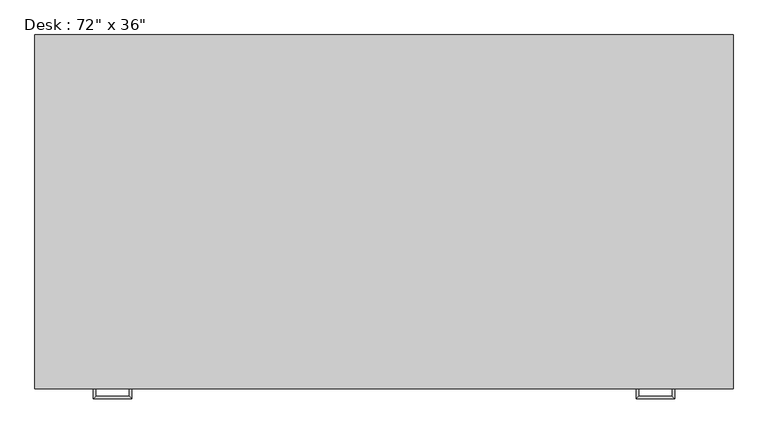
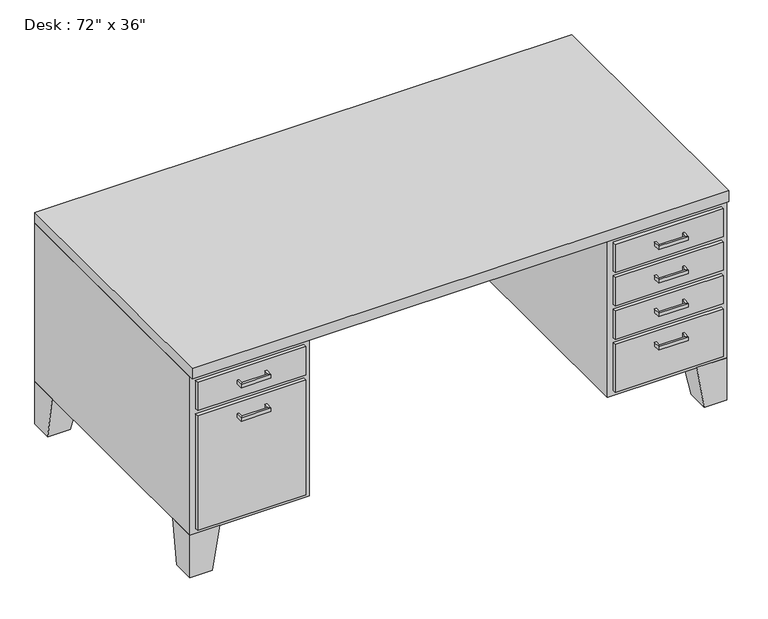
"""IFC4 building model written with IfcOpenShell, lengths in millimetres: furniture geometry."""

from ifc_helpers import new_model, si_unit, frame, origin, place, context, project, spatial, polyline, outline, extrude, faceted_brep, source, transform, mapped, element, save


def furniture_33f25304(model_context):
    return source(origin(), model_context, "Body", "SolidModel", [
        extrude(outline(polyline([(-133.35, -76.2), (234.95, -76.2), (234.95, -88.9), (-133.35, -88.9), (-133.35, -76.2)])), frame((0.0, 0.0, 603.25), z_axis=(0.0, 0.0, 1.0), x_axis=(1.0, 0.0, 0.0)), (0.0, 0.0, 1.0), 101.6),
        extrude(outline(polyline([(-133.35, -76.2), (234.95, -76.2), (234.95, -88.9), (-133.35, -88.9), (-133.35, -76.2)])), frame((0.0, 0.0, 171.45), z_axis=(0.0, 0.0, 1.0), x_axis=(1.0, 0.0, 0.0)), (0.0, 0.0, 1.0), 412.75),
        extrude(outline(polyline([(1289.05, -76.2), (1657.35, -76.2), (1657.35, -88.9), (1289.05, -88.9), (1289.05, -76.2)])), frame((0.0, 0.0, 603.25), z_axis=(0.0, 0.0, 1.0), x_axis=(1.0, 0.0, 0.0)), (0.0, 0.0, 1.0), 101.6),
        extrude(outline(polyline([(1289.05, -76.2), (1657.35, -76.2), (1657.35, -88.9), (1289.05, -88.9), (1289.05, -76.2)])), frame((0.0, 0.0, 171.45), z_axis=(0.0, 0.0, 1.0), x_axis=(1.0, 0.0, 0.0)), (0.0, 0.0, 1.0), 171.45),
        extrude(outline(polyline([(1289.05, -76.2), (1657.35, -76.2), (1657.35, -88.9), (1289.05, -88.9), (1289.05, -76.2)])), frame((0.0, 0.0, 482.6), z_axis=(0.0, 0.0, 1.0), x_axis=(1.0, 0.0, 0.0)), (0.0, 0.0, 1.0), 101.6),
        extrude(outline(polyline([(1289.05, -76.2), (1657.35, -76.2), (1657.35, -88.9), (1289.05, -88.9), (1289.05, -76.2)])), frame((0.0, 0.0, 361.95), z_axis=(0.0, 0.0, 1.0), x_axis=(1.0, 0.0, 0.0)), (0.0, 0.0, 1.0), 101.6),
        faceted_brep([(-50.8, -76.2, 152.4), (-50.8, 25.4, 152.4), (-152.4, 25.4, 152.4), (-152.4, -76.2, 152.4), (-76.2, -76.2, 0.0), (-152.4, -76.2, 0.0), (-152.4, 0.0, 0.0), (-76.2, 0.0, 0.0)], [[[0, 1, 2, 3]], [[4, 5, 6, 7]], [[4, 7, 1, 0]], [[7, 6, 2, 1]], [[6, 5, 3, 2]], [[5, 4, 0, 3]]]),
        faceted_brep([(-50.8, 838.2, 152.4), (-152.4, 838.2, 152.4), (-152.4, 736.6, 152.4), (-50.8, 736.6, 152.4), (-76.2, 838.2, 0.0), (-76.2, 762.0, 0.0), (-152.4, 762.0, 0.0), (-152.4, 838.2, 0.0)], [[[0, 1, 2, 3]], [[4, 5, 6, 7]], [[4, 7, 1, 0]], [[7, 6, 2, 1]], [[6, 5, 3, 2]], [[5, 4, 0, 3]]]),
        faceted_brep([(1574.8, 838.2, 152.4), (1574.8, 736.6, 152.4), (1676.4, 736.6, 152.4), (1676.4, 838.2, 152.4), (1600.2, 838.2, 0.0), (1676.4, 838.2, 0.0), (1676.4, 762.0, 0.0), (1600.2, 762.0, 0.0)], [[[0, 1, 2, 3]], [[4, 5, 6, 7]], [[4, 7, 1, 0]], [[7, 6, 2, 1]], [[6, 5, 3, 2]], [[5, 4, 0, 3]]]),
        faceted_brep([(1574.8, -76.2, 152.4), (1676.4, -76.2, 152.4), (1676.4, 25.4, 152.4), (1574.8, 25.4, 152.4), (1600.2, -76.2, 0.0), (1600.2, 0.0, 0.0), (1676.4, 0.0, 0.0), (1676.4, -76.2, 0.0)], [[[0, 1, 2, 3]], [[4, 5, 6, 7]], [[4, 7, 1, 0]], [[7, 6, 2, 1]], [[6, 5, 3, 2]], [[5, 4, 0, 3]]]),
        extrude(outline(polyline([(-152.4, -88.9), (-152.4, 838.2), (1676.4, 838.2), (1676.4, -88.9), (-152.4, -88.9)])), frame((0.0, 0.0, 723.9), z_axis=(0.0, 0.0, 1.0), x_axis=(1.0, 0.0, 0.0)), (0.0, 0.0, 1.0), 38.1),
        extrude(outline(polyline([(1270.0, -76.2), (1270.0, 711.2), (254.0, 711.2), (254.0, -76.2), (-152.4, -76.2), (-152.4, 838.2), (1676.4, 838.2), (1676.4, -76.2), (1270.0, -76.2)])), frame((0.0, 0.0, 152.4), z_axis=(0.0, 0.0, 1.0), x_axis=(1.0, 0.0, 0.0)), (0.0, 0.0, 1.0), 571.5),
        faceted_brep([(6.35, -88.9, 546.1), (6.35, -88.9, 533.4), (0.0, -88.9, 533.4), (0.0, -88.9, 546.1), (6.35, -107.95, 546.1), (6.35, -107.95, 533.4), (0.0, -114.3, 533.4), (0.0, -114.3, 546.1), (95.25, -107.95, 546.1), (95.25, -107.95, 533.4), (101.6, -114.3, 533.4), (101.6, -114.3, 546.1), (95.25, -88.9, 546.1), (101.6, -88.9, 546.1), (101.6, -88.9, 533.4), (95.25, -88.9, 533.4)], [[[0, 1, 2, 3]], [[1, 0, 4, 5]], [[2, 1, 5, 6]], [[3, 2, 6, 7]], [[0, 3, 7, 4]], [[5, 4, 8, 9]], [[6, 5, 9, 10]], [[7, 6, 10, 11]], [[4, 7, 11, 8]], [[12, 13, 14, 15]], [[9, 8, 12, 15]], [[10, 9, 15, 14]], [[11, 10, 14, 13]], [[8, 11, 13, 12]]]),
        faceted_brep([(6.35, -88.9, 666.75), (6.35, -88.9, 654.05), (0.0, -88.9, 654.05), (0.0, -88.9, 666.75), (6.35, -107.95, 666.75), (6.35, -107.95, 654.05), (0.0, -114.3, 654.05), (0.0, -114.3, 666.75), (95.25, -107.95, 666.75), (95.25, -107.95, 654.05), (101.6, -114.3, 654.05), (101.6, -114.3, 666.75), (95.25, -88.9, 666.75), (101.6, -88.9, 666.75), (101.6, -88.9, 654.05), (95.25, -88.9, 654.05)], [[[0, 1, 2, 3]], [[1, 0, 4, 5]], [[2, 1, 5, 6]], [[3, 2, 6, 7]], [[0, 3, 7, 4]], [[5, 4, 8, 9]], [[6, 5, 9, 10]], [[7, 6, 10, 11]], [[4, 7, 11, 8]], [[12, 13, 14, 15]], [[9, 8, 12, 15]], [[10, 9, 15, 14]], [[11, 10, 14, 13]], [[8, 11, 13, 12]]]),
        faceted_brep([(1517.65, -88.9, 304.8), (1524.0, -88.9, 304.8), (1524.0, -88.9, 292.1), (1517.65, -88.9, 292.1), (1517.65, -107.95, 304.8), (1524.0, -114.3, 304.8), (1524.0, -114.3, 292.1), (1517.65, -107.95, 292.1), (1428.75, -107.95, 304.8), (1422.4, -114.3, 304.8), (1422.4, -114.3, 292.1), (1428.75, -107.95, 292.1), (1428.75, -88.9, 304.8), (1428.75, -88.9, 292.1), (1422.4, -88.9, 292.1), (1422.4, -88.9, 304.8)], [[[0, 1, 2, 3]], [[1, 0, 4, 5]], [[2, 1, 5, 6]], [[3, 2, 6, 7]], [[0, 3, 7, 4]], [[5, 4, 8, 9]], [[6, 5, 9, 10]], [[7, 6, 10, 11]], [[4, 7, 11, 8]], [[12, 13, 14, 15]], [[9, 8, 12, 15]], [[10, 9, 15, 14]], [[11, 10, 14, 13]], [[8, 11, 13, 12]]]),
        faceted_brep([(1517.65, -88.9, 425.45), (1524.0, -88.9, 425.45), (1524.0, -88.9, 412.75), (1517.65, -88.9, 412.75), (1517.65, -107.95, 425.45), (1524.0, -114.3, 425.45), (1524.0, -114.3, 412.75), (1517.65, -107.95, 412.75), (1428.75, -107.95, 425.45), (1422.4, -114.3, 425.45), (1422.4, -114.3, 412.75), (1428.75, -107.95, 412.75), (1428.75, -88.9, 425.45), (1428.75, -88.9, 412.75), (1422.4, -88.9, 412.75), (1422.4, -88.9, 425.45)], [[[0, 1, 2, 3]], [[1, 0, 4, 5]], [[2, 1, 5, 6]], [[3, 2, 6, 7]], [[0, 3, 7, 4]], [[5, 4, 8, 9]], [[6, 5, 9, 10]], [[7, 6, 10, 11]], [[4, 7, 11, 8]], [[12, 13, 14, 15]], [[9, 8, 12, 15]], [[10, 9, 15, 14]], [[11, 10, 14, 13]], [[8, 11, 13, 12]]]),
        faceted_brep([(1517.65, -88.9, 546.1), (1524.0, -88.9, 546.1), (1524.0, -88.9, 533.4), (1517.65, -88.9, 533.4), (1517.65, -107.95, 546.1), (1524.0, -114.3, 546.1), (1524.0, -114.3, 533.4), (1517.65, -107.95, 533.4), (1428.75, -107.95, 546.1), (1422.4, -114.3, 546.1), (1422.4, -114.3, 533.4), (1428.75, -107.95, 533.4), (1428.75, -88.9, 546.1), (1428.75, -88.9, 533.4), (1422.4, -88.9, 533.4), (1422.4, -88.9, 546.1)], [[[0, 1, 2, 3]], [[1, 0, 4, 5]], [[2, 1, 5, 6]], [[3, 2, 6, 7]], [[0, 3, 7, 4]], [[5, 4, 8, 9]], [[6, 5, 9, 10]], [[7, 6, 10, 11]], [[4, 7, 11, 8]], [[12, 13, 14, 15]], [[9, 8, 12, 15]], [[10, 9, 15, 14]], [[11, 10, 14, 13]], [[8, 11, 13, 12]]]),
        faceted_brep([(1517.65, -88.9, 666.75), (1524.0, -88.9, 666.75), (1524.0, -88.9, 654.05), (1517.65, -88.9, 654.05), (1517.65, -107.95, 666.75), (1524.0, -114.3, 666.75), (1524.0, -114.3, 654.05), (1517.65, -107.95, 654.05), (1428.75, -107.95, 666.75), (1422.4, -114.3, 666.75), (1422.4, -114.3, 654.05), (1428.75, -107.95, 654.05), (1428.75, -88.9, 666.75), (1428.75, -88.9, 654.05), (1422.4, -88.9, 654.05), (1422.4, -88.9, 666.75)], [[[0, 1, 2, 3]], [[1, 0, 4, 5]], [[2, 1, 5, 6]], [[3, 2, 6, 7]], [[0, 3, 7, 4]], [[5, 4, 8, 9]], [[6, 5, 9, 10]], [[7, 6, 10, 11]], [[4, 7, 11, 8]], [[12, 13, 14, 15]], [[9, 8, 12, 15]], [[10, 9, 15, 14]], [[11, 10, 14, 13]], [[8, 11, 13, 12]]]),
    ])


if __name__ == "__main__":
    model = new_model("IFC4")
    model_context = context("Model", 3, world=origin())
    ifc_project = project(units=[si_unit("LENGTHUNIT", "METRE", prefix="MILLI")], contexts=[model_context])
    site = spatial("IfcSite", under=ifc_project)
    building = spatial("IfcBuilding", under=site)
    placement = place(None, origin())
    furniture_shape = furniture_33f25304(model_context)
    element("IfcFurniture", 1, ObjectType="Desk : 72\" x 36\"", at=placement, inside=building, context=model_context, shape_type="MappedRepresentation", body=[
        mapped(furniture_shape, transform((0.0, 0.0, 0.0), x_axis=(1.0, 0.0, 0.0), y_axis=(0.0, 1.0, 0.0), z_axis=(0.0, 0.0, 1.0))),
    ])
    save(model, "model.ifc")

# Revit data of these elements
# Type "Desk : 72\" x 36\""
#   Assembly Code = "E2020200"
#   Depth = 3' - 0"
#   Height = 2' - 6"
#   Leg Height = 0' - 6"
#   Width = 6' - 0"
#   Body Material = Laminate, Ivory, Matte
#   Handle/Leg Material = Steel, Chrome Plated
#   Top Material = Cherry
#   Default Elevation = 0
# Element 1 (IfcFurniture, "Desk : 72\" x 36\"")
#   Materials on its faces: "Steel, Chrome Plated", "Laminate, Ivory, Matte", "Cherry"
# Materials
#   "Laminate, Ivory, Matte": class "Plastic", colour RGB 247 247 239, transparency 0, Description = "Plastic Laminate - Ivory, Matte", Cost = 0
#   "Steel, Chrome Plated": class "Metal", colour RGB 17 17 17, transparency 0, Description = "Chromiuim plated steel", Cost = 0
#   "Cherry": class "Wood", colour RGB 226 177 128, transparency 0, Description = "Prunus Serotina", Cost = 0
